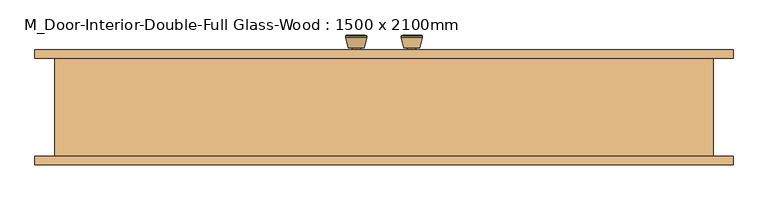
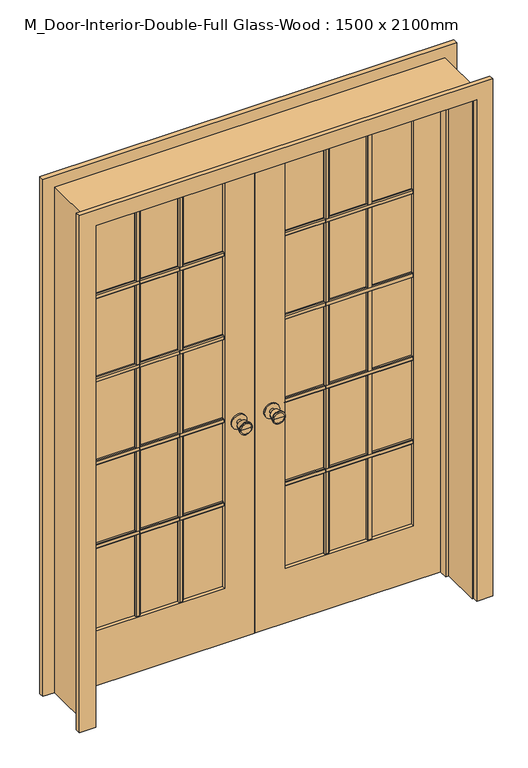
"""IFC4 building model written with IfcOpenShell, lengths in millimetres: door geometry, M_Door-Interior-Double-Full Glass-Wood : 1500 x 2100mm."""

from ifc_helpers import new_model, si_unit, point, frame, frame_2d, origin, place, context, project, spatial, polyline, circle_curve, trimmed, segment, composite_curve, outline, extrude, faceted_brep, source, transform, mapped, element, save
from ifc_brep_helpers import plane_surface, cylinder_surface, revolved_surface, advanced_brep


def m_door_interior_double_full_glass_wood_1500_x_2100mm_33705f2d(model_context):
    return source(origin(), model_context, "Body", "SolidModel", [
        advanced_brep(
        [(-65.0, 117.825, 914.4), (-75.0, 117.825, 914.4), (-55.0, 117.825, 914.4), (-85.4758676, 166.825, 914.4), (-65.0, 166.825, 914.4), (-44.5241324, 166.825, 914.4), (-90.0, 164.9971319, 914.4), (-40.0, 164.9971319, 914.4), (-90.0, 161.5334537, 914.4), (-40.0, 161.5334537, 914.4), (-83.636236, 136.825, 914.4), (-46.363764, 136.825, 914.4), (-75.0, 136.825, 914.4), (-55.0, 136.825, 914.4)],
        [
            (0, 1),
            (1, 2, circle_curve(frame((-65.0, 117.825, 914.4), z_axis=(0.0, -1.0, 0.0), x_axis=(1.0, 0.0, 0.0)), 10.0)),
            (2, 0),
            (2, 1, circle_curve(frame((-65.0, 117.825, 914.4), z_axis=(0.0, -1.0, 0.0), x_axis=(1.0, 0.0, 0.0)), 10.0)),
            (3, 4),
            (4, 5),
            (5, 3, circle_curve(frame((-65.0, 166.825, 914.4), z_axis=(0.0, 1.0, 0.0), x_axis=(1.0, 0.0, 0.0)), 20.4758676)),
            (3, 5, circle_curve(frame((-65.0, 166.825, 914.4), z_axis=(0.0, 1.0, 0.0), x_axis=(1.0, 0.0, 0.0)), 20.4758676)),
            (6, 3),
            (5, 7),
            (7, 6, circle_curve(frame((-65.0, 164.9971319, 914.4), z_axis=(0.0, 1.0, 0.0), x_axis=(1.0, 0.0, 0.0)), 25.0)),
            (6, 7, circle_curve(frame((-65.0, 164.9971319, 914.4), z_axis=(0.0, 1.0, 0.0), x_axis=(1.0, 0.0, 0.0)), 25.0)),
            (8, 6),
            (7, 9),
            (9, 8, circle_curve(frame((-65.0, 161.5334537, 914.4), z_axis=(0.0, 1.0, 0.0), x_axis=(1.0, 0.0, 0.0)), 25.0)),
            (8, 9, circle_curve(frame((-65.0, 161.5334537, 914.4), z_axis=(0.0, 1.0, 0.0), x_axis=(1.0, 0.0, 0.0)), 25.0)),
            (10, 8),
            (9, 11),
            (11, 10, circle_curve(frame((-65.0, 136.825, 914.4), z_axis=(0.0, 1.0, 0.0), x_axis=(1.0, 0.0, 0.0)), 18.636236)),
            (10, 11, circle_curve(frame((-65.0, 136.825, 914.4), z_axis=(0.0, 1.0, 0.0), x_axis=(1.0, 0.0, 0.0)), 18.636236)),
            (12, 10),
            (11, 13),
            (13, 12, circle_curve(frame((-65.0, 136.825, 914.4), z_axis=(0.0, 1.0, 0.0), x_axis=(1.0, 0.0, 0.0)), 10.0)),
            (12, 13, circle_curve(frame((-65.0, 136.825, 914.4), z_axis=(0.0, 1.0, 0.0), x_axis=(1.0, 0.0, 0.0)), 10.0)),
            (1, 12),
            (13, 2),
        ],
        [
            plane_surface(frame((-65.0, 117.825, 914.4), z_axis=(0.0, -1.0, 0.0), x_axis=(1.0, 0.0, 0.0))),
            plane_surface(frame((-65.0, 166.825, 914.4), z_axis=(0.0, 1.0, 0.0), x_axis=(1.0, 0.0, 0.0))),
            revolved_surface(polyline([(-44.5241324, 166.825, 914.4), (-40.0, 164.9971319, 914.4)]), (-65.0, 117.825, 914.4), (0.0, -1.0, 0.0)),
            cylinder_surface(frame((-65.0, 117.825, 914.4), z_axis=(0.0, -1.0, 0.0), x_axis=(1.0, 0.0, 0.0)), 25.0),
            revolved_surface(polyline([(-40.0, 161.5334537, 914.4), (-46.363764, 136.825, 914.4)]), (-65.0, 117.825, 914.4), (0.0, -1.0, 0.0)),
            plane_surface(frame((-65.0, 136.825, 914.4), z_axis=(0.0, -1.0, 0.0), x_axis=(1.0, 0.0, 0.0))),
            cylinder_surface(frame((-65.0, 117.825, 914.4), z_axis=(0.0, -1.0, 0.0), x_axis=(1.0, 0.0, 0.0)), 10.0),
        ],
        [
            (0, [[1, 2, 3]]),
            (0, [[-3, 4, -1]]),
            (1, [[5, 6, 7]]),
            (1, [[-6, -5, 8]]),
            (2, [[9, -7, 10, 11]]),
            (2, [[-10, -8, -9, 12]]),
            (3, [[13, -11, 14, 15]]),
            (3, [[-14, -12, -13, 16]]),
            (4, [[17, -15, 18, 19]]),
            (4, [[-18, -16, -17, 20]]),
            (5, [[21, -19, 22, 23]]),
            (5, [[-22, -20, -21, 24]]),
            (6, [[25, -23, 26, -2]]),
            (6, [[-26, -24, -25, -4]]),
        ],
    ),
        extrude(outline(composite_curve([segment(trimmed(circle_curve(frame_2d((914.4, -65.0)), 30.0), [point((914.4, -35.0))], [point((914.4, -95.0))], False, "CARTESIAN"), True, "CONTINUOUS"), segment(trimmed(circle_curve(frame_2d((914.4, -65.0)), 30.0), [point((914.4, -95.0))], [point((914.4, -35.0))], False, "CARTESIAN"), True, "CONTINUOUS")], self_intersect=False)), frame((0.0, 111.825, 0.0), z_axis=(0.0, 1.0, 0.0), x_axis=(0.0, 0.0, 1.0)), (0.0, 0.0, 1.0), 6.0),
        advanced_brep(
        [(-65.0, 70.825, 914.4), (-55.0, 70.825, 914.4), (-75.0, 70.825, 914.4), (-85.4758676, 21.825, 914.4), (-44.5241324, 21.825, 914.4), (-65.0, 21.825, 914.4), (-90.0, 23.6528681, 914.4), (-40.0, 23.6528681, 914.4), (-90.0, 27.1165463, 914.4), (-40.0, 27.1165463, 914.4), (-83.636236, 51.825, 914.4), (-46.363764, 51.825, 914.4), (-75.0, 51.825, 914.4), (-55.0, 51.825, 914.4)],
        [
            (0, 1),
            (1, 2, circle_curve(frame((-65.0, 70.825, 914.4), z_axis=(0.0, 1.0, 0.0), x_axis=(1.0, 0.0, 0.0)), 10.0)),
            (2, 0),
            (2, 1, circle_curve(frame((-65.0, 70.825, 914.4), z_axis=(0.0, 1.0, 0.0), x_axis=(1.0, 0.0, 0.0)), 10.0)),
            (3, 4, circle_curve(frame((-65.0, 21.825, 914.4), z_axis=(0.0, -1.0, 0.0), x_axis=(1.0, 0.0, 0.0)), 20.4758676)),
            (4, 5),
            (5, 3),
            (4, 3, circle_curve(frame((-65.0, 21.825, 914.4), z_axis=(0.0, -1.0, 0.0), x_axis=(1.0, 0.0, 0.0)), 20.4758676)),
            (6, 7, circle_curve(frame((-65.0, 23.6528681, 914.4), z_axis=(0.0, -1.0, 0.0), x_axis=(1.0, 0.0, 0.0)), 25.0)),
            (7, 4),
            (3, 6),
            (7, 6, circle_curve(frame((-65.0, 23.6528681, 914.4), z_axis=(0.0, -1.0, 0.0), x_axis=(1.0, 0.0, 0.0)), 25.0)),
            (8, 9, circle_curve(frame((-65.0, 27.1165463, 914.4), z_axis=(0.0, -1.0, 0.0), x_axis=(1.0, 0.0, 0.0)), 25.0)),
            (9, 7),
            (6, 8),
            (9, 8, circle_curve(frame((-65.0, 27.1165463, 914.4), z_axis=(0.0, -1.0, 0.0), x_axis=(1.0, 0.0, 0.0)), 25.0)),
            (10, 11, circle_curve(frame((-65.0, 51.825, 914.4), z_axis=(0.0, -1.0, 0.0), x_axis=(1.0, 0.0, 0.0)), 18.636236)),
            (11, 9),
            (8, 10),
            (11, 10, circle_curve(frame((-65.0, 51.825, 914.4), z_axis=(0.0, -1.0, 0.0), x_axis=(1.0, 0.0, 0.0)), 18.636236)),
            (12, 13, circle_curve(frame((-65.0, 51.825, 914.4), z_axis=(0.0, -1.0, 0.0), x_axis=(1.0, 0.0, 0.0)), 10.0)),
            (13, 11),
            (10, 12),
            (13, 12, circle_curve(frame((-65.0, 51.825, 914.4), z_axis=(0.0, -1.0, 0.0), x_axis=(1.0, 0.0, 0.0)), 10.0)),
            (1, 13),
            (12, 2),
        ],
        [
            plane_surface(frame((-65.0, 70.825, 914.4), z_axis=(0.0, 1.0, 0.0), x_axis=(1.0, 0.0, 0.0))),
            plane_surface(frame((-65.0, 21.825, 914.4), z_axis=(0.0, -1.0, 0.0), x_axis=(1.0, 0.0, 0.0))),
            revolved_surface(polyline([(-44.5241324, 21.825, 914.4), (-40.0, 23.6528681, 914.4)]), (-65.0, 70.825, 914.4), (0.0, 1.0, 0.0)),
            cylinder_surface(frame((-65.0, 70.825, 914.4), z_axis=(0.0, 1.0, 0.0), x_axis=(1.0, 0.0, 0.0)), 25.0),
            revolved_surface(polyline([(-40.0, 27.1165463, 914.4), (-46.363764, 51.825, 914.4)]), (-65.0, 70.825, 914.4), (0.0, 1.0, 0.0)),
            plane_surface(frame((-65.0, 51.825, 914.4), z_axis=(0.0, 1.0, 0.0), x_axis=(1.0, 0.0, 0.0))),
            cylinder_surface(frame((-65.0, 70.825, 914.4), z_axis=(0.0, 1.0, 0.0), x_axis=(1.0, 0.0, 0.0)), 10.0),
        ],
        [
            (0, [[1, 2, 3]]),
            (0, [[-3, 4, -1]]),
            (1, [[5, 6, 7]]),
            (1, [[8, -7, -6]]),
            (2, [[9, 10, -5, 11]]),
            (2, [[12, -11, -8, -10]]),
            (3, [[13, 14, -9, 15]]),
            (3, [[16, -15, -12, -14]]),
            (4, [[17, 18, -13, 19]]),
            (4, [[20, -19, -16, -18]]),
            (5, [[21, 22, -17, 23]]),
            (5, [[24, -23, -20, -22]]),
            (6, [[-2, 25, -21, 26]]),
            (6, [[-4, -26, -24, -25]]),
        ],
    ),
        extrude(outline(composite_curve([segment(trimmed(circle_curve(frame_2d((914.4, -65.0)), 30.0), [point((914.4, -35.0))], [point((914.4, -95.0))], False, "CARTESIAN"), True, "CONTINUOUS"), segment(trimmed(circle_curve(frame_2d((914.4, -65.0)), 30.0), [point((914.4, -95.0))], [point((914.4, -35.0))], False, "CARTESIAN"), True, "CONTINUOUS")], self_intersect=False)), frame((0.0, 70.825, 0.0), z_axis=(0.0, 1.0, 0.0), x_axis=(0.0, 0.0, 1.0)), (0.0, 0.0, 1.0), 6.0),
        extrude(outline(polyline([(90.825, 1639.525), (90.825, 1620.475), (84.475, 1620.475), (81.3, 1623.65), (81.3, 1636.35), (84.475, 1639.525), (90.825, 1639.525)])), frame((120.0, 0.0, 0.0), z_axis=(1.0, 0.0, 0.0), x_axis=(0.0, 1.0, 0.0)), (0.0, 0.0, 1.0), 510.0),
        extrude(outline(polyline([(90.825, 1289.525), (90.825, 1270.475), (84.475, 1270.475), (81.3, 1273.65), (81.3, 1286.35), (84.475, 1289.525), (90.825, 1289.525)])), frame((120.0, 0.0, 0.0), z_axis=(1.0, 0.0, 0.0), x_axis=(0.0, 1.0, 0.0)), (0.0, 0.0, 1.0), 510.0),
        extrude(outline(polyline([(90.825, 939.525), (90.825, 920.475), (84.475, 920.475), (81.3, 923.65), (81.3, 936.35), (84.475, 939.525), (90.825, 939.525)])), frame((120.0, 0.0, 0.0), z_axis=(1.0, 0.0, 0.0), x_axis=(0.0, 1.0, 0.0)), (0.0, 0.0, 1.0), 510.0),
        extrude(outline(polyline([(90.825, 589.525), (90.825, 570.475), (84.475, 570.475), (81.3, 573.65), (81.3, 586.35), (84.475, 589.525), (90.825, 589.525)])), frame((120.0, 0.0, 0.0), z_axis=(1.0, 0.0, 0.0), x_axis=(0.0, 1.0, 0.0)), (0.0, 0.0, 1.0), 510.0),
        extrude(outline(polyline([(450.475, 90.825), (469.525, 90.825), (469.525, 84.475), (466.35, 81.3), (453.65, 81.3), (450.475, 84.475), (450.475, 90.825)])), frame((0.0, 0.0, 230.0), z_axis=(0.0, 0.0, 1.0), x_axis=(1.0, 0.0, 0.0)), (0.0, 0.0, 1.0), 1750.0),
        extrude(outline(polyline([(280.475, 90.825), (299.525, 90.825), (299.525, 84.475), (296.35, 81.3), (283.65, 81.3), (280.475, 84.475), (280.475, 90.825)])), frame((0.0, 0.0, 230.0), z_axis=(0.0, 0.0, 1.0), x_axis=(1.0, 0.0, 0.0)), (0.0, 0.0, 1.0), 1750.0),
        extrude(outline(polyline([(97.825, 1639.525), (104.175, 1639.525), (107.35, 1636.35), (107.35, 1623.65), (104.175, 1620.475), (97.825, 1620.475), (97.825, 1639.525)])), frame((-630.0, 0.0, 0.0), z_axis=(1.0, 0.0, 0.0), x_axis=(0.0, 1.0, 0.0)), (0.0, 0.0, 1.0), 510.0),
        extrude(outline(polyline([(97.825, 1289.525), (104.175, 1289.525), (107.35, 1286.35), (107.35, 1273.65), (104.175, 1270.475), (97.825, 1270.475), (97.825, 1289.525)])), frame((-630.0, 0.0, 0.0), z_axis=(1.0, 0.0, 0.0), x_axis=(0.0, 1.0, 0.0)), (0.0, 0.0, 1.0), 510.0),
        extrude(outline(polyline([(97.825, 939.525), (104.175, 939.525), (107.35, 936.35), (107.35, 923.65), (104.175, 920.475), (97.825, 920.475), (97.825, 939.525)])), frame((-630.0, 0.0, 0.0), z_axis=(1.0, 0.0, 0.0), x_axis=(0.0, 1.0, 0.0)), (0.0, 0.0, 1.0), 510.0),
        extrude(outline(polyline([(97.825, 589.525), (104.175, 589.525), (107.35, 586.35), (107.35, 573.65), (104.175, 570.475), (97.825, 570.475), (97.825, 589.525)])), frame((-630.0, 0.0, 0.0), z_axis=(1.0, 0.0, 0.0), x_axis=(0.0, 1.0, 0.0)), (0.0, 0.0, 1.0), 510.0),
        extrude(outline(polyline([(-299.525, 97.825), (-299.525, 104.175), (-296.35, 107.35), (-283.65, 107.35), (-280.475, 104.175), (-280.475, 97.825), (-299.525, 97.825)])), frame((0.0, 0.0, 230.0), z_axis=(0.0, 0.0, 1.0), x_axis=(1.0, 0.0, 0.0)), (0.0, 0.0, 1.0), 1750.0),
        extrude(outline(polyline([(-469.525, 97.825), (-469.525, 104.175), (-466.35, 107.35), (-453.65, 107.35), (-450.475, 104.175), (-450.475, 97.825), (-469.525, 97.825)])), frame((0.0, 0.0, 230.0), z_axis=(0.0, 0.0, 1.0), x_axis=(1.0, 0.0, 0.0)), (0.0, 0.0, 1.0), 1750.0),
        extrude(outline(polyline([(97.825, 1639.525), (104.175, 1639.525), (107.35, 1636.35), (107.35, 1623.65), (104.175, 1620.475), (97.825, 1620.475), (97.825, 1639.525)])), frame((120.0, 0.0, 0.0), z_axis=(1.0, 0.0, 0.0), x_axis=(0.0, 1.0, 0.0)), (0.0, 0.0, 1.0), 510.0),
        extrude(outline(polyline([(97.825, 1289.525), (104.175, 1289.525), (107.35, 1286.35), (107.35, 1273.65), (104.175, 1270.475), (97.825, 1270.475), (97.825, 1289.525)])), frame((120.0, 0.0, 0.0), z_axis=(1.0, 0.0, 0.0), x_axis=(0.0, 1.0, 0.0)), (0.0, 0.0, 1.0), 510.0),
        extrude(outline(polyline([(97.825, 939.525), (104.175, 939.525), (107.35, 936.35), (107.35, 923.65), (104.175, 920.475), (97.825, 920.475), (97.825, 939.525)])), frame((120.0, 0.0, 0.0), z_axis=(1.0, 0.0, 0.0), x_axis=(0.0, 1.0, 0.0)), (0.0, 0.0, 1.0), 510.0),
        extrude(outline(polyline([(97.825, 589.525), (104.175, 589.525), (107.35, 586.35), (107.35, 573.65), (104.175, 570.475), (97.825, 570.475), (97.825, 589.525)])), frame((120.0, 0.0, 0.0), z_axis=(1.0, 0.0, 0.0), x_axis=(0.0, 1.0, 0.0)), (0.0, 0.0, 1.0), 510.0),
        extrude(outline(polyline([(450.475, 97.825), (450.475, 104.175), (453.65, 107.35), (466.35, 107.35), (469.525, 104.175), (469.525, 97.825), (450.475, 97.825)])), frame((0.0, 0.0, 230.0), z_axis=(0.0, 0.0, 1.0), x_axis=(1.0, 0.0, 0.0)), (0.0, 0.0, 1.0), 1750.0),
        extrude(outline(polyline([(280.475, 97.825), (280.475, 104.175), (283.65, 107.35), (296.35, 107.35), (299.525, 104.175), (299.525, 97.825), (280.475, 97.825)])), frame((0.0, 0.0, 230.0), z_axis=(0.0, 0.0, 1.0), x_axis=(1.0, 0.0, 0.0)), (0.0, 0.0, 1.0), 1750.0),
        extrude(outline(polyline([(90.825, 1639.525), (90.825, 1620.475), (84.475, 1620.475), (81.3, 1623.65), (81.3, 1636.35), (84.475, 1639.525), (90.825, 1639.525)])), frame((-630.0, 0.0, 0.0), z_axis=(1.0, 0.0, 0.0), x_axis=(0.0, 1.0, 0.0)), (0.0, 0.0, 1.0), 510.0),
        extrude(outline(polyline([(90.825, 1289.525), (90.825, 1270.475), (84.475, 1270.475), (81.3, 1273.65), (81.3, 1286.35), (84.475, 1289.525), (90.825, 1289.525)])), frame((-630.0, 0.0, 0.0), z_axis=(1.0, 0.0, 0.0), x_axis=(0.0, 1.0, 0.0)), (0.0, 0.0, 1.0), 510.0),
        extrude(outline(polyline([(90.825, 939.525), (90.825, 920.475), (84.475, 920.475), (81.3, 923.65), (81.3, 936.35), (84.475, 939.525), (90.825, 939.525)])), frame((-630.0, 0.0, 0.0), z_axis=(1.0, 0.0, 0.0), x_axis=(0.0, 1.0, 0.0)), (0.0, 0.0, 1.0), 510.0),
        extrude(outline(polyline([(90.825, 589.525), (90.825, 570.475), (84.475, 570.475), (81.3, 573.65), (81.3, 586.35), (84.475, 589.525), (90.825, 589.525)])), frame((-630.0, 0.0, 0.0), z_axis=(1.0, 0.0, 0.0), x_axis=(0.0, 1.0, 0.0)), (0.0, 0.0, 1.0), 510.0),
        extrude(outline(polyline([(-299.525, 90.825), (-280.475, 90.825), (-280.475, 84.475), (-283.65, 81.3), (-296.35, 81.3), (-299.525, 84.475), (-299.525, 90.825)])), frame((0.0, 0.0, 230.0), z_axis=(0.0, 0.0, 1.0), x_axis=(1.0, 0.0, 0.0)), (0.0, 0.0, 1.0), 1750.0),
        extrude(outline(polyline([(-469.525, 90.825), (-450.475, 90.825), (-450.475, 84.475), (-453.65, 81.3), (-466.35, 81.3), (-469.525, 84.475), (-469.525, 90.825)])), frame((0.0, 0.0, 230.0), z_axis=(0.0, 0.0, 1.0), x_axis=(1.0, 0.0, 0.0)), (0.0, 0.0, 1.0), 1750.0),
        advanced_brep(
        [(65.0, 70.825, 914.4), (75.0, 70.825, 914.4), (55.0, 70.825, 914.4), (85.4758676, 21.825, 914.4), (65.0, 21.825, 914.4), (44.5241324, 21.825, 914.4), (90.0, 23.6528681, 914.4), (40.0, 23.6528681, 914.4), (90.0, 27.1165463, 914.4), (40.0, 27.1165463, 914.4), (83.636236, 51.825, 914.4), (46.363764, 51.825, 914.4), (75.0, 51.825, 914.4), (55.0, 51.825, 914.4)],
        [
            (0, 1),
            (1, 2, circle_curve(frame((65.0, 70.825, 914.4), z_axis=(0.0, 1.0, 0.0), x_axis=(-1.0, 0.0, 0.0)), 10.0)),
            (2, 0),
            (2, 1, circle_curve(frame((65.0, 70.825, 914.4), z_axis=(0.0, 1.0, 0.0), x_axis=(-1.0, 0.0, 0.0)), 10.0)),
            (3, 4),
            (4, 5),
            (5, 3, circle_curve(frame((65.0, 21.825, 914.4), z_axis=(0.0, -1.0, 0.0), x_axis=(-1.0, 0.0, 0.0)), 20.4758676)),
            (3, 5, circle_curve(frame((65.0, 21.825, 914.4), z_axis=(0.0, -1.0, 0.0), x_axis=(-1.0, 0.0, 0.0)), 20.4758676)),
            (6, 3),
            (5, 7),
            (7, 6, circle_curve(frame((65.0, 23.6528681, 914.4), z_axis=(0.0, -1.0, 0.0), x_axis=(-1.0, 0.0, 0.0)), 25.0)),
            (6, 7, circle_curve(frame((65.0, 23.6528681, 914.4), z_axis=(0.0, -1.0, 0.0), x_axis=(-1.0, 0.0, 0.0)), 25.0)),
            (8, 6),
            (7, 9),
            (9, 8, circle_curve(frame((65.0, 27.1165463, 914.4), z_axis=(0.0, -1.0, 0.0), x_axis=(-1.0, 0.0, 0.0)), 25.0)),
            (8, 9, circle_curve(frame((65.0, 27.1165463, 914.4), z_axis=(0.0, -1.0, 0.0), x_axis=(-1.0, 0.0, 0.0)), 25.0)),
            (10, 8),
            (9, 11),
            (11, 10, circle_curve(frame((65.0, 51.825, 914.4), z_axis=(0.0, -1.0, 0.0), x_axis=(-1.0, 0.0, 0.0)), 18.636236)),
            (10, 11, circle_curve(frame((65.0, 51.825, 914.4), z_axis=(0.0, -1.0, 0.0), x_axis=(-1.0, 0.0, 0.0)), 18.636236)),
            (12, 10),
            (11, 13),
            (13, 12, circle_curve(frame((65.0, 51.825, 914.4), z_axis=(0.0, -1.0, 0.0), x_axis=(-1.0, 0.0, 0.0)), 10.0)),
            (12, 13, circle_curve(frame((65.0, 51.825, 914.4), z_axis=(0.0, -1.0, 0.0), x_axis=(-1.0, 0.0, 0.0)), 10.0)),
            (1, 12),
            (13, 2),
        ],
        [
            plane_surface(frame((65.0, 70.825, 914.4), z_axis=(0.0, 1.0, 0.0), x_axis=(-1.0, 0.0, 0.0))),
            plane_surface(frame((65.0, 21.825, 914.4), z_axis=(0.0, -1.0, 0.0), x_axis=(-1.0, 0.0, 0.0))),
            revolved_surface(polyline([(44.5241324, 21.825, 914.4), (40.0, 23.6528681, 914.4)]), (65.0, 70.825, 914.4), (0.0, 1.0, 0.0)),
            cylinder_surface(frame((65.0, 70.825, 914.4), z_axis=(0.0, 1.0, 0.0), x_axis=(-1.0, 0.0, 0.0)), 25.0),
            revolved_surface(polyline([(40.0, 27.1165463, 914.4), (46.363764, 51.825, 914.4)]), (65.0, 70.825, 914.4), (0.0, 1.0, 0.0)),
            plane_surface(frame((65.0, 51.825, 914.4), z_axis=(0.0, 1.0, 0.0), x_axis=(-1.0, 0.0, 0.0))),
            cylinder_surface(frame((65.0, 70.825, 914.4), z_axis=(0.0, 1.0, 0.0), x_axis=(-1.0, 0.0, 0.0)), 10.0),
        ],
        [
            (0, [[1, 2, 3]]),
            (0, [[-3, 4, -1]]),
            (1, [[5, 6, 7]]),
            (1, [[-6, -5, 8]]),
            (2, [[9, -7, 10, 11]]),
            (2, [[-10, -8, -9, 12]]),
            (3, [[13, -11, 14, 15]]),
            (3, [[-14, -12, -13, 16]]),
            (4, [[17, -15, 18, 19]]),
            (4, [[-18, -16, -17, 20]]),
            (5, [[21, -19, 22, 23]]),
            (5, [[-22, -20, -21, 24]]),
            (6, [[25, -23, 26, -2]]),
            (6, [[-26, -24, -25, -4]]),
        ],
    ),
        extrude(outline(composite_curve([segment(trimmed(circle_curve(frame_2d((914.4, 65.0)), 30.0), [point((914.4, 35.0))], [point((914.4, 95.0))], False, "CARTESIAN"), True, "CONTINUOUS"), segment(trimmed(circle_curve(frame_2d((914.4, 65.0)), 30.0), [point((914.4, 95.0))], [point((914.4, 35.0))], False, "CARTESIAN"), True, "CONTINUOUS")], self_intersect=False)), frame((0.0, 70.825, 0.0), z_axis=(0.0, 1.0, 0.0), x_axis=(0.0, 0.0, 1.0)), (0.0, 0.0, 1.0), 6.0),
        advanced_brep(
        [(65.0, 117.825, 914.4), (55.0, 117.825, 914.4), (75.0, 117.825, 914.4), (85.4758676, 166.825, 914.4), (44.5241324, 166.825, 914.4), (65.0, 166.825, 914.4), (90.0, 164.9971319, 914.4), (40.0, 164.9971319, 914.4), (90.0, 161.5334537, 914.4), (40.0, 161.5334537, 914.4), (83.636236, 136.825, 914.4), (46.363764, 136.825, 914.4), (75.0, 136.825, 914.4), (55.0, 136.825, 914.4)],
        [
            (0, 1),
            (1, 2, circle_curve(frame((65.0, 117.825, 914.4), z_axis=(0.0, -1.0, 0.0), x_axis=(-1.0, 0.0, 0.0)), 10.0)),
            (2, 0),
            (2, 1, circle_curve(frame((65.0, 117.825, 914.4), z_axis=(0.0, -1.0, 0.0), x_axis=(-1.0, 0.0, 0.0)), 10.0)),
            (3, 4, circle_curve(frame((65.0, 166.825, 914.4), z_axis=(0.0, 1.0, 0.0), x_axis=(-1.0, 0.0, 0.0)), 20.4758676)),
            (4, 5),
            (5, 3),
            (4, 3, circle_curve(frame((65.0, 166.825, 914.4), z_axis=(0.0, 1.0, 0.0), x_axis=(-1.0, 0.0, 0.0)), 20.4758676)),
            (6, 7, circle_curve(frame((65.0, 164.9971319, 914.4), z_axis=(0.0, 1.0, 0.0), x_axis=(-1.0, 0.0, 0.0)), 25.0)),
            (7, 4),
            (3, 6),
            (7, 6, circle_curve(frame((65.0, 164.9971319, 914.4), z_axis=(0.0, 1.0, 0.0), x_axis=(-1.0, 0.0, 0.0)), 25.0)),
            (8, 9, circle_curve(frame((65.0, 161.5334537, 914.4), z_axis=(0.0, 1.0, 0.0), x_axis=(-1.0, 0.0, 0.0)), 25.0)),
            (9, 7),
            (6, 8),
            (9, 8, circle_curve(frame((65.0, 161.5334537, 914.4), z_axis=(0.0, 1.0, 0.0), x_axis=(-1.0, 0.0, 0.0)), 25.0)),
            (10, 11, circle_curve(frame((65.0, 136.825, 914.4), z_axis=(0.0, 1.0, 0.0), x_axis=(-1.0, 0.0, 0.0)), 18.636236)),
            (11, 9),
            (8, 10),
            (11, 10, circle_curve(frame((65.0, 136.825, 914.4), z_axis=(0.0, 1.0, 0.0), x_axis=(-1.0, 0.0, 0.0)), 18.636236)),
            (12, 13, circle_curve(frame((65.0, 136.825, 914.4), z_axis=(0.0, 1.0, 0.0), x_axis=(-1.0, 0.0, 0.0)), 10.0)),
            (13, 11),
            (10, 12),
            (13, 12, circle_curve(frame((65.0, 136.825, 914.4), z_axis=(0.0, 1.0, 0.0), x_axis=(-1.0, 0.0, 0.0)), 10.0)),
            (1, 13),
            (12, 2),
        ],
        [
            plane_surface(frame((65.0, 117.825, 914.4), z_axis=(0.0, -1.0, 0.0), x_axis=(-1.0, 0.0, 0.0))),
            plane_surface(frame((65.0, 166.825, 914.4), z_axis=(0.0, 1.0, 0.0), x_axis=(-1.0, 0.0, 0.0))),
            revolved_surface(polyline([(44.5241324, 166.825, 914.4), (40.0, 164.9971319, 914.4)]), (65.0, 117.825, 914.4), (0.0, -1.0, 0.0)),
            cylinder_surface(frame((65.0, 117.825, 914.4), z_axis=(0.0, -1.0, 0.0), x_axis=(-1.0, 0.0, 0.0)), 25.0),
            revolved_surface(polyline([(40.0, 161.5334537, 914.4), (46.363764, 136.825, 914.4)]), (65.0, 117.825, 914.4), (0.0, -1.0, 0.0)),
            plane_surface(frame((65.0, 136.825, 914.4), z_axis=(0.0, -1.0, 0.0), x_axis=(-1.0, 0.0, 0.0))),
            cylinder_surface(frame((65.0, 117.825, 914.4), z_axis=(0.0, -1.0, 0.0), x_axis=(-1.0, 0.0, 0.0)), 10.0),
        ],
        [
            (0, [[1, 2, 3]]),
            (0, [[-3, 4, -1]]),
            (1, [[5, 6, 7]]),
            (1, [[8, -7, -6]]),
            (2, [[9, 10, -5, 11]]),
            (2, [[12, -11, -8, -10]]),
            (3, [[13, 14, -9, 15]]),
            (3, [[16, -15, -12, -14]]),
            (4, [[17, 18, -13, 19]]),
            (4, [[20, -19, -16, -18]]),
            (5, [[21, 22, -17, 23]]),
            (5, [[24, -23, -20, -22]]),
            (6, [[-2, 25, -21, 26]]),
            (6, [[-4, -26, -24, -25]]),
        ],
    ),
        extrude(outline(composite_curve([segment(trimmed(circle_curve(frame_2d((914.4, 65.0)), 30.0), [point((914.4, 35.0))], [point((914.4, 95.0))], False, "CARTESIAN"), True, "CONTINUOUS"), segment(trimmed(circle_curve(frame_2d((914.4, 65.0)), 30.0), [point((914.4, 95.0))], [point((914.4, 35.0))], False, "CARTESIAN"), True, "CONTINUOUS")], self_intersect=False)), frame((0.0, 111.825, 0.0), z_axis=(0.0, 1.0, 0.0), x_axis=(0.0, 0.0, 1.0)), (0.0, 0.0, 1.0), 6.0),
        extrude(outline(polyline([(0.0, 756.35), (0.0, 821.35), (2171.35, 821.35), (2171.35, -821.35), (0.0, -821.35), (0.0, -756.35), (2106.35, -756.35), (2106.35, 756.35), (0.0, 756.35)])), frame((0.0, 111.825, 0.0), z_axis=(0.0, 1.0, 0.0), x_axis=(0.0, 0.0, 1.0)), (0.0, 0.0, 1.0), 20.0),
        extrude(outline(polyline([(0.0, 756.35), (0.0, 821.35), (2171.35, 821.35), (2171.35, -821.35), (0.0, -821.35), (0.0, -756.35), (2106.35, -756.35), (2106.35, 756.35), (0.0, 756.35)])), frame((0.0, -138.175, 0.0), z_axis=(0.0, 1.0, 0.0), x_axis=(0.0, 0.0, 1.0)), (0.0, 0.0, 1.0), 20.0),
        extrude(outline(polyline([(2100.0, -750.0), (0.0, -750.0), (0.0, -1.6019111), (2100.0, -1.6019111), (2100.0, -750.0)]), holes=[polyline([(230.0, -630.0), (1980.0, -630.0), (1980.0, -120.0), (230.0, -120.0), (230.0, -630.0)])]), frame((0.0, 76.825, 0.0), z_axis=(0.0, 1.0, 0.0), x_axis=(0.0, 0.0, 1.0)), (0.0, 0.0, 1.0), 35.0),
        extrude(outline(polyline([(0.0, 750.0), (2100.0, 750.0), (2100.0, 1.5875), (0.0, 1.5875), (0.0, 750.0)]), holes=[polyline([(1980.0, 120.0), (1980.0, 630.0), (230.0, 630.0), (230.0, 120.0), (1980.0, 120.0)])]), frame((0.0, 76.825, 0.0), z_axis=(0.0, 1.0, 0.0), x_axis=(0.0, 0.0, 1.0)), (0.0, 0.0, 1.0), 35.0),
        faceted_brep([(775.0, 111.825, 0.0), (775.0, -118.175, 0.0), (750.0, -118.175, 0.0), (750.0, 41.9, 0.0), (737.3, 41.9, 0.0), (737.3, 76.825, 0.0), (750.0, 76.825, 0.0), (750.0, 111.825, 0.0), (775.0, 111.825, 2125.0), (775.0, -118.175, 2125.0), (-775.0, -118.175, 2125.0), (-775.0, -118.175, 0.0), (-750.0, -118.175, 0.0), (-750.0, -118.175, 2100.0), (750.0, -118.175, 2100.0), (750.0, 41.9, 2100.0), (-750.0, 41.9, 2100.0), (-750.0, 41.9, 0.0), (-737.3, 41.9, 0.0), (-737.3, 41.9, 2087.3), (737.3, 41.9, 2087.3), (737.3, 76.825, 2087.3), (1.5875, 76.825, 2087.3), (-1.6019111, 76.825, 2087.3), (-737.3, 76.825, 2087.3), (-737.3, 76.825, 0.0), (-750.0, 76.825, 0.0), (-750.0, 76.825, 2100.0), (-1.6019111, 76.825, 2100.0), (1.5875, 76.825, 2100.0), (750.0, 76.825, 2100.0), (750.0, 111.825, 2100.0), (1.5875, 111.825, 2100.0), (-1.6019111, 111.825, 2100.0), (-750.0, 111.825, 2100.0), (-750.0, 111.825, 0.0), (-775.0, 111.825, 0.0), (-775.0, 111.825, 2125.0)], [[[0, 1, 2, 3, 4, 5, 6, 7]], [[1, 0, 8, 9]], [[2, 1, 9, 10, 11, 12, 13, 14]], [[3, 2, 14, 15]], [[4, 3, 15, 16, 17, 18, 19, 20]], [[5, 4, 20, 21]], [[6, 5, 21, 22, 23, 24, 25, 26, 27, 28, 29, 30]], [[7, 6, 30, 31]], [[0, 7, 31, 32, 33, 34, 35, 36, 37, 8]], [[9, 8, 37, 10]], [[14, 13, 16, 15]], [[20, 19, 24, 23, 22, 21]], [[31, 30, 29, 28, 27, 34, 33, 32]], [[12, 11, 36, 35, 26, 25, 18, 17]], [[11, 10, 37, 36]], [[13, 12, 17, 16]], [[19, 18, 25, 24]], [[27, 26, 35, 34]]]),
        extrude(outline(polyline([(630.0, 90.825), (120.0, 90.825), (120.0, 97.825), (630.0, 97.825), (630.0, 90.825)])), frame((0.0, 0.0, 230.0), z_axis=(0.0, 0.0, 1.0), x_axis=(1.0, 0.0, 0.0)), (0.0, 0.0, 1.0), 1750.0),
        extrude(outline(polyline([(-120.0, 90.825), (-630.0, 90.825), (-630.0, 97.825), (-120.0, 97.825), (-120.0, 90.825)])), frame((0.0, 0.0, 230.0), z_axis=(0.0, 0.0, 1.0), x_axis=(1.0, 0.0, 0.0)), (0.0, 0.0, 1.0), 1750.0),
    ])


if __name__ == "__main__":
    model = new_model("IFC4")
    model_context = context("Model", 3, world=origin())
    ifc_project = project(units=[si_unit("LENGTHUNIT", "METRE", prefix="MILLI")], contexts=[model_context])
    site = spatial("IfcSite", under=ifc_project)
    building = spatial("IfcBuilding", under=site)
    placement = place(None, origin())
    m_door_interior_double_full_glass_wood_1500_x_2100mm_shape = m_door_interior_double_full_glass_wood_1500_x_2100mm_33705f2d(model_context)
    element("IfcDoor", 1, ObjectType="M_Door-Interior-Double-Full Glass-Wood : 1500 x 2100mm", at=placement, inside=building, context=model_context, shape_type="MappedRepresentation", body=[
        mapped(m_door_interior_double_full_glass_wood_1500_x_2100mm_shape, transform((0.0, 0.0, 0.0), x_axis=(1.0, 0.0, 0.0), y_axis=(0.0, 1.0, 0.0), z_axis=(0.0, 0.0, 1.0))),
    ])
    save(model, "model.ifc")

# Revit data of these elements
# Type "M_Door-Interior-Double-Full Glass-Wood : 1500 x 2100mm"
#   Type Mark = "49"
#   Assembly Code = "C1020300"
#   Analytic Construction = "French door, wood frame with single glass"
#   Top Rail = 12 cm
#   Thickness = 3.5 cm
#   Thermal Resistance (R) = 0.188367 (m²·K)/W
#   Swing Angle [instance default] = 90.00°
#   Stiles = 12 cm
#   Rough Width = 155 cm
#   Rough Height = 212.5 cm
#   Panel Width = 75 cm
#   Height = 210 cm
#   Width = 150 cm
#   Heat Transfer Coefficient (U) = 5.30918 W/(m²·K)
#   Bottom Rail = 23 cm
#   Show Grill [instance default] = yes
#   Trim Material = Cherry
#   Panel Material = Cherry
#   Frame Material = Cherry
#   Door Handle Material = Aluminum
#   Visual Light Transmittance = 0
#   Solar Heat Gain Coefficient = 0
#   Wall Closure = (empty or 0)
#   Function = (empty or 0)
# Element 1 (IfcDoor, "M_Door-Interior-Double-Full Glass-Wood : 1500 x 2100mm")
#   Materials on its faces: "Cherry", "Aluminum", "Glass"
# Materials
#   "Cherry": class "Wood", colour RGB 226 177 128, transparency 0, Description = "Prunus Serotina", Cost = 0
#   "Aluminum": class "Metal", colour RGB 247 247 247, transparency 0, Description = "Aluminum 6061", Cost = 0
#   "Glass": class "Glass", colour RGB 0 128 192, transparency 0.9, Description = "Soda Lime Glass", Cost = 0
